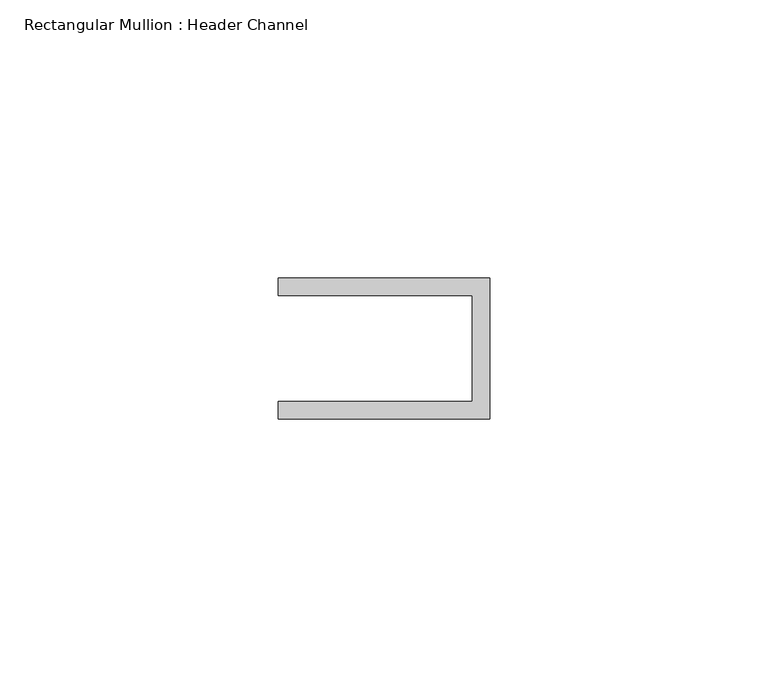
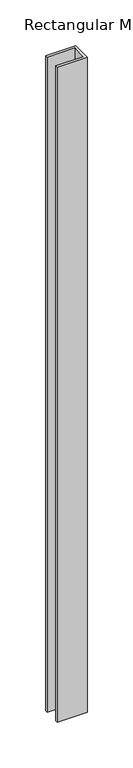
"""IFC4 building model written with IfcOpenShell, lengths in millimetres: member geometry, Rectangular Mullion : Header Channel."""

from ifc_helpers import new_model, si_unit, frame, origin, place, context, project, spatial, polyline, outline, extrude, source, transform, mapped, element, save


def rectangular_mullion_header_channel_2e6e9d6b(model_context):
    return source(origin(), model_context, "Body", "SweptSolid", [
        extrude(outline(polyline([(0.0, 12.7), (0.0, -12.7), (-38.1, -12.7), (-38.1, -9.525), (-3.175, -9.525), (-3.175, 9.525), (-38.1, 9.525), (-38.1, 12.7), (0.0, 12.7)])), frame((0.0, 0.0, -876.6174999), z_axis=(0.0, 0.0, 1.0), x_axis=(1.0, 0.0, 0.0)), (0.0, 0.0, 1.0), 876.6174999),
    ])


if __name__ == "__main__":
    model = new_model("IFC4")
    model_context = context("Model", 3, world=origin())
    ifc_project = project(units=[si_unit("LENGTHUNIT", "METRE", prefix="MILLI")], contexts=[model_context])
    site = spatial("IfcSite", under=ifc_project)
    building = spatial("IfcBuilding", under=site)
    placement = place(None, origin())
    rectangular_mullion_header_channel_shape = rectangular_mullion_header_channel_2e6e9d6b(model_context)
    element("IfcMember", 1, ObjectType="Rectangular Mullion : Header Channel", at=placement, inside=building, context=model_context, shape_type="MappedRepresentation", body=[
        mapped(rectangular_mullion_header_channel_shape, transform((0.0, 0.0, 0.0), x_axis=(1.0, 0.0, 0.0), y_axis=(0.0, 1.0, 0.0), z_axis=(0.0, 0.0, 1.0))),
    ])
    save(model, "model.ifc")

# Revit data of these elements
# Type "Rectangular Mullion : Header Channel"
#   built-in parameter 1007322 = 0.0833333 (stored number, unit not read)
#   built-in parameter 1007321 = -0.03125 (stored number, unit not read)
#   built-in parameter 1007320 = 0.0416667 (stored number, unit not read)
# Element 1 (IfcMember, "Rectangular Mullion : Header Channel")
#   Materials on its faces: "ALUM"
# Materials
#   "ALUM": class "Generic", colour RGB 157 157 157, transparency 0, Cost = 0
